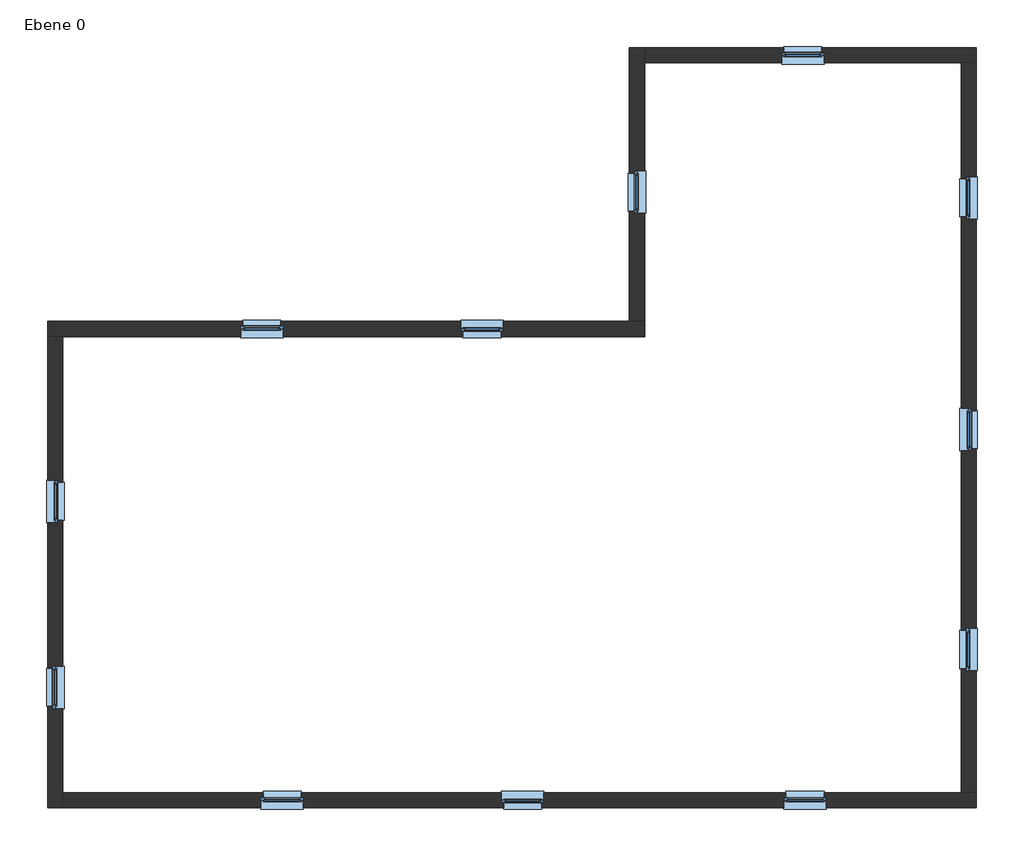
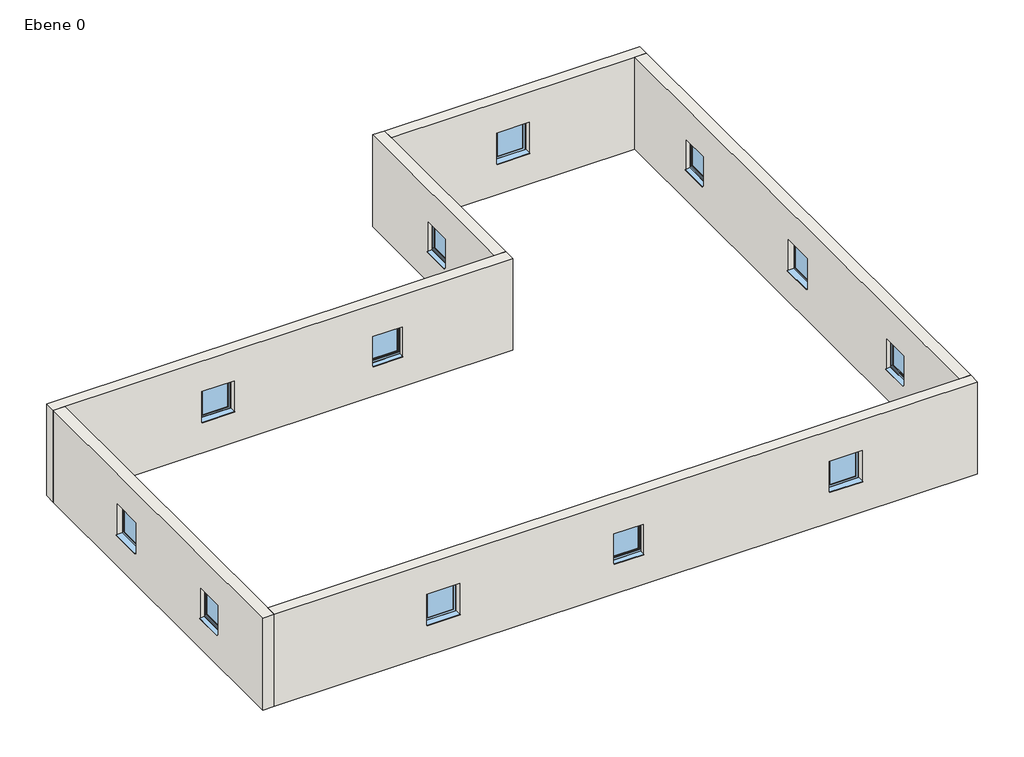
# One storey: 12 windows, 6 walls.
"""IFC4 building model written with IfcOpenShell, lengths in millimetres."""

import ifcopenshell
import ifcopenshell.guid

model = None  # the IFC model being written
_history = None  # IfcOwnerHistory: only IFC2X3 demands one
_inside = {}  # id of a spatial element -> (the spatial element, [elements in it])
_under = {}  # id of a project, library or spatial element -> (it, [spatial elements below it])
_declared = {}  # id of a project -> (the project, [libraries it declares])
_typed = {}  # id of a type object -> (the type object, [elements of that type])
_made_of = {}  # id of a material, layer set ... -> (it, [elements and type objects made of it])


def new_model(schema):
    """Start an empty IFC model of exactly this schema.

    Asked for "IFC4X3", IfcOpenShell would pick the latest addendum, in which some entities
    have other attributes; the version numbers below select the first issue.
    IFC2X3 requires an IfcOwnerHistory on every rooted entity: one is made here for all.
    """
    global model, _history
    if schema == "IFC4X3":
        model = ifcopenshell.file(schema_version=(4, 3, 0, 0))
    else:
        model = ifcopenshell.file(schema=schema)
    _inside.clear()
    _under.clear()
    _declared.clear()
    _typed.clear()
    _made_of.clear()
    _history = None
    if model.schema == "IFC2X3":
        org = make("IfcOrganization", Name="unknown")
        user = make(
            "IfcPersonAndOrganization",
            ThePerson=make("IfcPerson", FamilyName="unknown"),
            TheOrganization=org,
        )
        app = make(
            "IfcApplication",
            ApplicationDeveloper=org,
            Version="unknown",
            ApplicationFullName="unknown",
            ApplicationIdentifier="unknown",
        )
        _history = make(
            "IfcOwnerHistory",
            OwningUser=user,
            OwningApplication=app,
            ChangeAction="ADDED",
            CreationDate=0,
        )
    return model


def make(cls, **values):
    """One entity of the class cls with the attributes given. An attribute that is None is left unset."""
    return model.create_entity(
        cls, **{name: value for name, value in values.items() if value is not None}
    )


def rooted(cls, **values):
    """An entity with a GlobalId (a new one), such as an element, a storey or a relation."""
    return make(cls, GlobalId=ifcopenshell.guid.new(), OwnerHistory=_history, **values)


def si_unit(unit_type, name, prefix=None):
    """IfcSIUnit, for example si_unit("LENGTHUNIT", "METRE", prefix="MILLI")."""
    return make("IfcSIUnit", UnitType=unit_type, Prefix=prefix, Name=name)


def assignment(units):
    """IfcUnitAssignment: the units of a project."""
    return None if units is None else make("IfcUnitAssignment", Units=units)


def point(xyz):
    """IfcCartesianPoint."""
    return None if xyz is None else make("IfcCartesianPoint", Coordinates=xyz)


def direction(xyz):
    """IfcDirection."""
    return None if xyz is None else make("IfcDirection", DirectionRatios=xyz)


def frame(location, z_axis=None, x_axis=None):
    """IfcAxis2Placement3D, a coordinate frame: its origin and axes. An axis left out is left unset."""
    return make(
        "IfcAxis2Placement3D",
        Location=point(location),
        Axis=direction(z_axis),
        RefDirection=direction(x_axis),
    )


def origin():
    """The frame at (0, 0, 0) with its axes left unset."""
    return frame((0.0, 0.0, 0.0))


def place(relative_to, where):
    """IfcLocalPlacement: puts the frame where relative to a parent placement (None: the world)."""
    return make(
        "IfcLocalPlacement", PlacementRelTo=relative_to, RelativePlacement=where
    )


def context(
    kind, dimensions, precision=None, world=None, true_north=None, identifier=None
):
    """IfcGeometricRepresentationContext, for example the 3D "Model" context."""
    return make(
        "IfcGeometricRepresentationContext",
        ContextIdentifier=identifier,
        ContextType=kind,
        CoordinateSpaceDimension=dimensions,
        Precision=precision,
        WorldCoordinateSystem=world,
        TrueNorth=true_north,
    )


def project(units=None, contexts=None):
    """IfcProject with its units and contexts."""
    return rooted(
        "IfcProject",
        Name="project",
        RepresentationContexts=contexts,
        UnitsInContext=assignment(units),
    )


def spatial(cls, under=None, at=None, **own):
    """A site, building, storey or space (cls), placed at a placement, below another one or the project."""
    s = rooted(cls, ObjectPlacement=at, **own)
    if under is not None:
        _under.setdefault(under.id(), (under, []))[1].append(s)
    return s


def polyline(points):
    """IfcPolyline through the points."""
    return make("IfcPolyline", Points=[point(p) for p in points])


def outline(outer, holes=None, kind="AREA"):
    """IfcArbitraryClosedProfileDef: a profile drawn as a closed curve; with holes, ...WithVoids."""
    if holes is None:
        return make("IfcArbitraryClosedProfileDef", ProfileType=kind, OuterCurve=outer)
    return make(
        "IfcArbitraryProfileDefWithVoids",
        ProfileType=kind,
        OuterCurve=outer,
        InnerCurves=holes,
    )


def extrude(swept, where, along, depth):
    """IfcExtrudedAreaSolid: the profile swept, set in the frame where, extruded along a direction by depth."""
    return make(
        "IfcExtrudedAreaSolid",
        SweptArea=swept,
        Position=where,
        ExtrudedDirection=direction(along),
        Depth=depth,
    )


def faces_of(points, faces, orient=None, outer=None):
    """IfcFace entities. A face is a list of loops; a loop is a list of indices into points, from 0.

    orient and outer hold one flag for each loop. By default every Orientation is true, the
    first loop of a face is its IfcFaceOuterBound and the others are IfcFaceBound.
    """
    made = []
    for i, loops in enumerate(faces):
        bounds = []
        for j, loop in enumerate(loops):
            is_outer = j == 0 if outer is None else outer[i][j]
            bounds.append(
                make(
                    "IfcFaceOuterBound" if is_outer else "IfcFaceBound",
                    Bound=make("IfcPolyLoop", Polygon=[points[k] for k in loop]),
                    Orientation=True if orient is None else orient[i][j],
                )
            )
        made.append(make("IfcFace", Bounds=bounds))
    return made


def faceted_brep(points, faces, orient=None, outer=None, voids=None):
    """IfcFacetedBrep: a solid bounded by flat faces; with voids (closed shells), ...WithVoids."""
    shared = [point(p) for p in points]
    hull = make("IfcClosedShell", CfsFaces=faces_of(shared, faces, orient, outer))
    if voids is None:
        return make("IfcFacetedBrep", Outer=hull)
    return make(
        "IfcFacetedBrepWithVoids",
        Outer=hull,
        Voids=[
            make(cls, CfsFaces=faces_of(shared, fs, o, b)) for cls, fs, o, b in voids
        ],
    )


def shape(context_of_items, identifier, shape_type, items):
    """IfcShapeRepresentation: the items that make up one representation, for example the "Body"."""
    return make(
        "IfcShapeRepresentation",
        ContextOfItems=context_of_items,
        RepresentationIdentifier=identifier,
        RepresentationType=shape_type,
        Items=items,
    )


def source(mapping_origin, context_of_items, identifier, shape_type, items):
    """IfcRepresentationMap: a shape defined once, which mapped items show again and again."""
    return make(
        "IfcRepresentationMap",
        MappingOrigin=mapping_origin,
        MappedRepresentation=shape(context_of_items, identifier, shape_type, items),
    )


def transform(
    local_origin,
    x_axis=None,
    y_axis=None,
    z_axis=None,
    scale=None,
    scale2=None,
    scale3=None,
    uniform=True,
):
    """IfcCartesianTransformationOperator3D, or its non-uniform kind. x_axis, y_axis, z_axis: its Axis1, 2, 3."""
    if uniform:
        return make(
            "IfcCartesianTransformationOperator3D",
            Axis1=direction(x_axis),
            Axis2=direction(y_axis),
            LocalOrigin=point(local_origin),
            Scale=scale,
            Axis3=direction(z_axis),
        )
    return make(
        "IfcCartesianTransformationOperator3DnonUniform",
        Axis1=direction(x_axis),
        Axis2=direction(y_axis),
        LocalOrigin=point(local_origin),
        Scale=scale,
        Axis3=direction(z_axis),
        Scale2=scale2,
        Scale3=scale3,
    )


def mapped(mapping_source, mapping_target):
    """IfcMappedItem: shows the shape of a source again, moved by a transform."""
    return make(
        "IfcMappedItem", MappingSource=mapping_source, MappingTarget=mapping_target
    )


def made_of(thing, what):
    """Note that an element or type object is made of a material, layer set ...; save() writes the relation."""
    if what is not None:
        _made_of.setdefault(what.id(), (what, []))[1].append(thing)
    return thing


def element(
    cls,
    number,
    at=None,
    inside=None,
    cuts=None,
    type_object=None,
    material=None,
    context=None,
    identifier="Body",
    shape_type=None,
    held_by="IfcProductDefinitionShape",
    body=None,
    shapes=None,
    **own,
):
    """One element of the class cls, such as IfcWall. Its Tag is "e" and its number.

    at: its placement. inside: the storey or other place that contains it. cuts: it is an
    opening in that element (IfcRelVoidsElement). A single representation is given by context,
    identifier, shape_type and body (its items); several are given by shapes. held_by: the class
    of the entity that holds the representations. save() writes the other relations.
    """
    e = rooted(cls, Tag="e%d" % number, ObjectPlacement=at, **own)
    if body is not None:
        shapes = [shape(context, identifier, shape_type, body)]
    if shapes is not None:
        e.Representation = make(held_by, Representations=shapes)
    if inside is not None:
        _inside.setdefault(inside.id(), (inside, []))[1].append(e)
    if cuts is not None:
        rooted(
            "IfcRelVoidsElement", RelatingBuildingElement=cuts, RelatedOpeningElement=e
        )
    if type_object is not None:
        _typed.setdefault(type_object.id(), (type_object, []))[1].append(e)
    return made_of(e, material)


def aggregate(whole, parts):
    """IfcRelAggregates: a whole, such as a stair, and the parts it consists of."""
    return rooted("IfcRelAggregates", RelatingObject=whole, RelatedObjects=parts)


def save(model, path):
    """Write the relations noted so far, then the file.

    IfcRelAggregates (storeys below a building ...), IfcRelContainedInSpatialStructure (elements
    in a storey), IfcRelDefinesByType, IfcRelAssociatesMaterial and IfcRelDeclares: one each for
    every whole, place, type object, material and project.
    """
    for whole, parts in _under.values():
        aggregate(whole, parts)
    for where, things in _inside.values():
        rooted(
            "IfcRelContainedInSpatialStructure",
            RelatedElements=things,
            RelatingStructure=where,
        )
    for kind, things in _typed.values():
        rooted("IfcRelDefinesByType", RelatedObjects=things, RelatingType=kind)
    for what, things in _made_of.values():
        rooted("IfcRelAssociatesMaterial", RelatedObjects=things, RelatingMaterial=what)
    for by, libraries in _declared.values():
        rooted("IfcRelDeclares", RelatingContext=by, RelatedDefinitions=libraries)
    model.write(path)


def window_1_01_x_1_01_b7243dc8(model_context):
    return source(origin(), model_context, "Body", "SolidModel", [
        extrude(outline(polyline([(-525.0, -210.0), (-525.0, 0.0), (485.0, 0.0), (485.0, -210.0), (-525.0, -210.0)])), frame((0.0, 0.0, 1005.0), z_axis=(0.0, 0.0, 1.0), x_axis=(1.0, 0.0, 0.0)), (0.0, 0.0, 1.0), 15.0),
        extrude(outline(polyline([(375.0, -15.0), (-415.0, -15.0), (-415.0, 15.0), (375.0, 15.0), (375.0, -15.0)])), frame((0.0, 0.0, 1110.0), z_axis=(0.0, 0.0, 1.0), x_axis=(1.0, 0.0, 0.0)), (0.0, 0.0, 1.0), 790.0),
        extrude(outline(polyline([(70.0221543, 1020.0), (210.0, 1000.0), (210.0, 990.0), (208.0, 990.0), (208.0, 998.3604634), (69.8240723, 1018.0), (60.0, 1018.0), (60.0, 1020.0), (70.0221543, 1020.0)])), frame((-475.0, 0.0, 0.0), z_axis=(1.0, 0.0, 0.0), x_axis=(0.0, 1.0, 0.0)), (0.0, 0.0, 1.0), 910.0),
        extrude(outline(polyline([(2010.0, 485.0), (2010.0, -525.0), (1000.0, -525.0), (1000.0, 485.0), (2010.0, 485.0)]), holes=[polyline([(1930.0, 405.0), (1080.0, 405.0), (1080.0, -445.0), (1930.0, -445.0), (1930.0, 405.0)])]), frame((0.0, 0.0, 0.0), z_axis=(0.0, 1.0, 0.0), x_axis=(0.0, 0.0, 1.0)), (0.0, 0.0, 1.0), 60.0),
        faceted_brep([(435.0, 0.0, 1960.0), (435.0, -30.0, 1960.0), (435.0, -30.0, 1050.0), (435.0, 0.0, 1050.0), (-475.0, -30.0, 1960.0), (-475.0, -30.0, 1050.0), (375.0, -30.0, 1110.0), (-415.0, -30.0, 1110.0), (-415.0, -30.0, 1900.0), (375.0, -30.0, 1900.0), (-475.0, 0.0, 1050.0), (-475.0, 0.0, 1960.0), (405.0, 0.0, 1930.0), (-445.0, 0.0, 1930.0), (-445.0, 0.0, 1080.0), (405.0, 0.0, 1080.0), (405.0, 30.0, 1930.0), (405.0, 30.0, 1080.0), (-445.0, 30.0, 1080.0), (-445.0, 30.0, 1930.0), (375.0, 30.0, 1900.0), (-415.0, 30.0, 1900.0), (-415.0, 30.0, 1110.0), (375.0, 30.0, 1110.0)], [[[0, 1, 2, 3]], [[1, 4, 5, 2], [6, 7, 8, 9]], [[3, 2, 5, 10]], [[3, 10, 11, 0], [12, 13, 14, 15]], [[16, 12, 15, 17]], [[17, 15, 14, 18]], [[17, 18, 19, 16], [20, 21, 22, 23]], [[9, 20, 23, 6]], [[6, 23, 22, 7]], [[10, 5, 4, 11]], [[18, 14, 13, 19]], [[7, 22, 21, 8]], [[11, 4, 1, 0]], [[19, 13, 12, 16]], [[8, 21, 20, 9]]]),
    ])


model = new_model("IFC4")

# Units and contexts
model_context = context("Model", 3, world=origin())
ifc_project = project(units=[si_unit("LENGTHUNIT", "METRE", prefix="MILLI")], contexts=[model_context])

# Site, building, storey
site = spatial("IfcSite", under=ifc_project)
building = spatial("IfcBuilding", under=site)
storey = spatial("IfcBuildingStorey", under=building, Name="Ebene 0", Elevation=0.0)

# Walls
placement = place(None, origin())
element("IfcWall", 1, ObjectType="MW 24.0 WD 12.0", at=placement, inside=storey, context=model_context, shape_type="Brep", body=[
    faceted_brep([(-13369.6797169, 6985.6067473, 0.0), (-13009.6797169, 6985.6067473, 0.0), (810.3202831, 6985.6067473, 0.0), (810.3202831, 6985.6067473, 3000.0), (-13009.6797169, 6985.6067473, 3000.0), (-13369.6797169, 6985.6067473, 3000.0), (-3509.6797169, 6985.6067473, 1960.0), (-2599.6797169, 6985.6067473, 1960.0), (-2599.6797169, 6985.6067473, 1000.0), (-3509.6797169, 6985.6067473, 1000.0), (-7779.6797169, 6985.6067473, 1000.0), (-8789.6797169, 6985.6067473, 1000.0), (-8789.6797169, 6985.6067473, 2010.0), (-7779.6797169, 6985.6067473, 2010.0), (-13369.6797169, 7345.6067473, 0.0), (-13369.6797169, 7345.6067473, 3000.0), (450.3202831, 7345.6067473, 3000.0), (810.3202831, 7345.6067473, 3000.0), (810.3202831, 7345.6067473, 0.0), (450.3202831, 7345.6067473, 0.0), (-3559.6797169, 7345.6067473, 1000.0), (-2549.6797169, 7345.6067473, 1000.0), (-2549.6797169, 7345.6067473, 2010.0), (-3559.6797169, 7345.6067473, 2010.0), (-7829.6797169, 7345.6067473, 1960.0), (-8739.6797169, 7345.6067473, 1960.0), (-8739.6797169, 7345.6067473, 1000.0), (-7829.6797169, 7345.6067473, 1000.0), (-3509.6797169, 7105.6067473, 1960.0), (-2599.6797169, 7105.6067473, 1960.0), (-2599.6797169, 7105.6067473, 1000.0), (-3509.6797169, 7105.6067473, 1000.0), (-2549.6797169, 7105.6067473, 1000.0), (-3559.6797169, 7105.6067473, 1000.0), (-2549.6797169, 7105.6067473, 2010.0), (-3559.6797169, 7105.6067473, 2010.0), (-7829.6797169, 7225.6067473, 1960.0), (-8739.6797169, 7225.6067473, 1960.0), (-8739.6797169, 7225.6067473, 1000.0), (-7829.6797169, 7225.6067473, 1000.0), (-8789.6797169, 7225.6067473, 1000.0), (-7779.6797169, 7225.6067473, 1000.0), (-8789.6797169, 7225.6067473, 2010.0), (-7779.6797169, 7225.6067473, 2010.0)], [[[0, 1, 2, 3, 4, 5], [6, 7, 8, 9], [10, 11, 12, 13]], [[14, 15, 16, 17, 18, 19], [20, 21, 22, 23], [24, 25, 26, 27]], [[2, 1, 0, 14, 19, 18]], [[5, 4, 3, 17, 16, 15]], [[0, 5, 15, 14]], [[3, 2, 18, 17]], [[6, 28, 29, 7]], [[7, 29, 30, 8]], [[28, 6, 9, 31]], [[8, 30, 32, 21, 20, 33, 31, 9]], [[34, 35, 23, 22]], [[35, 33, 20, 23]], [[35, 34, 32, 30, 29, 28, 31, 33]], [[32, 34, 22, 21]], [[24, 36, 37, 25]], [[25, 37, 38, 26]], [[36, 24, 27, 39]], [[26, 38, 40, 11, 10, 41, 39, 27]], [[42, 43, 13, 12]], [[43, 41, 10, 13]], [[43, 42, 40, 38, 37, 36, 39, 41]], [[40, 42, 12, 11]]]),
])
element("IfcWall", 2, ObjectType="MW 24.0 WD 12.0", at=placement, inside=storey, context=model_context, shape_type="Brep", body=[
    faceted_brep([(-13009.6797169, -4214.3932527, 0.0), (-13009.6797169, -3854.3932527, 0.0), (-13009.6797169, 6985.6067473, 0.0), (-13009.6797169, 6985.6067473, 3000.0), (-13009.6797169, -3854.3932527, 3000.0), (-13009.6797169, -4214.3932527, 3000.0), (-13009.6797169, -844.3932527, 1000.0), (-13009.6797169, -1854.3932527, 1000.0), (-13009.6797169, -1854.3932527, 2010.0), (-13009.6797169, -844.3932527, 2010.0), (-13009.6797169, 2615.6067473, 1960.0), (-13009.6797169, 3525.6067473, 1960.0), (-13009.6797169, 3525.6067473, 1000.0), (-13009.6797169, 2615.6067473, 1000.0), (-13369.6797169, -4214.3932527, 0.0), (-13369.6797169, -4214.3932527, 3000.0), (-13369.6797169, 6985.6067473, 3000.0), (-13369.6797169, 6985.6067473, 0.0), (-13369.6797169, -894.3932527, 1960.0), (-13369.6797169, -1804.3932527, 1960.0), (-13369.6797169, -1804.3932527, 1000.0), (-13369.6797169, -894.3932527, 1000.0), (-13369.6797169, 2565.6067473, 1000.0), (-13369.6797169, 3575.6067473, 1000.0), (-13369.6797169, 3575.6067473, 2010.0), (-13369.6797169, 2565.6067473, 2010.0), (-13249.6797169, -894.3932527, 1960.0), (-13249.6797169, -1804.3932527, 1960.0), (-13249.6797169, -1804.3932527, 1000.0), (-13249.6797169, -894.3932527, 1000.0), (-13249.6797169, -1854.3932527, 1000.0), (-13249.6797169, -844.3932527, 1000.0), (-13249.6797169, -1854.3932527, 2010.0), (-13249.6797169, -844.3932527, 2010.0), (-13129.6797169, 2615.6067473, 1960.0), (-13129.6797169, 3525.6067473, 1960.0), (-13129.6797169, 3525.6067473, 1000.0), (-13129.6797169, 2615.6067473, 1000.0), (-13129.6797169, 3575.6067473, 1000.0), (-13129.6797169, 2565.6067473, 1000.0), (-13129.6797169, 3575.6067473, 2010.0), (-13129.6797169, 2565.6067473, 2010.0)], [[[0, 1, 2, 3, 4, 5], [6, 7, 8, 9], [10, 11, 12, 13]], [[14, 15, 16, 17], [18, 19, 20, 21], [22, 23, 24, 25]], [[2, 1, 0, 14, 17]], [[5, 4, 3, 16, 15]], [[0, 5, 15, 14]], [[3, 2, 17, 16]], [[18, 26, 27, 19]], [[19, 27, 28, 20]], [[26, 18, 21, 29]], [[20, 28, 30, 7, 6, 31, 29, 21]], [[32, 33, 9, 8]], [[33, 31, 6, 9]], [[33, 32, 30, 28, 27, 26, 29, 31]], [[30, 32, 8, 7]], [[10, 34, 35, 11]], [[11, 35, 36, 12]], [[34, 10, 13, 37]], [[12, 36, 38, 23, 22, 39, 37, 13]], [[40, 41, 25, 24]], [[41, 39, 22, 25]], [[41, 40, 38, 36, 35, 34, 37, 39]], [[38, 40, 24, 23]]]),
])
element("IfcWall", 3, ObjectType="MW 24.0 WD 12.0", at=placement, inside=storey, context=model_context, shape_type="Brep", body=[
    faceted_brep([(8690.3202831, -3854.3932527, 0.0), (8330.3202831, -3854.3932527, 0.0), (-13009.6797169, -3854.3932527, 0.0), (-13009.6797169, -3854.3932527, 3000.0), (8330.3202831, -3854.3932527, 3000.0), (8690.3202831, -3854.3932527, 3000.0), (5080.3202831, -3854.3932527, 1960.0), (4170.3202831, -3854.3932527, 1960.0), (4170.3202831, -3854.3932527, 1000.0), (5080.3202831, -3854.3932527, 1000.0), (-2589.6797169, -3854.3932527, 1000.0), (-1579.6797169, -3854.3932527, 1000.0), (-1579.6797169, -3854.3932527, 2010.0), (-2589.6797169, -3854.3932527, 2010.0), (-7344.6797169, -3854.3932527, 1960.0), (-8254.6797169, -3854.3932527, 1960.0), (-8254.6797169, -3854.3932527, 1000.0), (-7344.6797169, -3854.3932527, 1000.0), (8690.3202831, -4214.3932527, 0.0), (8690.3202831, -4214.3932527, 3000.0), (-13009.6797169, -4214.3932527, 3000.0), (-13009.6797169, -4214.3932527, 0.0), (5130.3202831, -4214.3932527, 1000.0), (4120.3202831, -4214.3932527, 1000.0), (4120.3202831, -4214.3932527, 2010.0), (5130.3202831, -4214.3932527, 2010.0), (-2539.6797169, -4214.3932527, 1960.0), (-1629.6797169, -4214.3932527, 1960.0), (-1629.6797169, -4214.3932527, 1000.0), (-2539.6797169, -4214.3932527, 1000.0), (-7294.6797169, -4214.3932527, 1000.0), (-8304.6797169, -4214.3932527, 1000.0), (-8304.6797169, -4214.3932527, 2010.0), (-7294.6797169, -4214.3932527, 2010.0), (5080.3202831, -3974.3932527, 1960.0), (4170.3202831, -3974.3932527, 1960.0), (4170.3202831, -3974.3932527, 1000.0), (5080.3202831, -3974.3932527, 1000.0), (4120.3202831, -3974.3932527, 1000.0), (5130.3202831, -3974.3932527, 1000.0), (4120.3202831, -3974.3932527, 2010.0), (5130.3202831, -3974.3932527, 2010.0), (-2539.6797169, -4094.3932527, 1960.0), (-1629.6797169, -4094.3932527, 1960.0), (-1629.6797169, -4094.3932527, 1000.0), (-2539.6797169, -4094.3932527, 1000.0), (-1579.6797169, -4094.3932527, 1000.0), (-2589.6797169, -4094.3932527, 1000.0), (-1579.6797169, -4094.3932527, 2010.0), (-2589.6797169, -4094.3932527, 2010.0), (-7344.6797169, -3974.3932527, 1960.0), (-8254.6797169, -3974.3932527, 1960.0), (-8254.6797169, -3974.3932527, 1000.0), (-7344.6797169, -3974.3932527, 1000.0), (-8304.6797169, -3974.3932527, 1000.0), (-7294.6797169, -3974.3932527, 1000.0), (-8304.6797169, -3974.3932527, 2010.0), (-7294.6797169, -3974.3932527, 2010.0)], [[[0, 1, 2, 3, 4, 5], [6, 7, 8, 9], [10, 11, 12, 13], [14, 15, 16, 17]], [[18, 19, 20, 21], [22, 23, 24, 25], [26, 27, 28, 29], [30, 31, 32, 33]], [[2, 1, 0, 18, 21]], [[5, 4, 3, 20, 19]], [[0, 5, 19, 18]], [[3, 2, 21, 20]], [[6, 34, 35, 7]], [[7, 35, 36, 8]], [[34, 6, 9, 37]], [[8, 36, 38, 23, 22, 39, 37, 9]], [[40, 41, 25, 24]], [[41, 39, 22, 25]], [[41, 40, 38, 36, 35, 34, 37, 39]], [[38, 40, 24, 23]], [[26, 42, 43, 27]], [[27, 43, 44, 28]], [[42, 26, 29, 45]], [[28, 44, 46, 11, 10, 47, 45, 29]], [[48, 49, 13, 12]], [[49, 47, 10, 13]], [[49, 48, 46, 44, 43, 42, 45, 47]], [[46, 48, 12, 11]], [[14, 50, 51, 15]], [[15, 51, 52, 16]], [[50, 14, 17, 53]], [[16, 52, 54, 31, 30, 55, 53, 17]], [[56, 57, 33, 32]], [[57, 55, 30, 33]], [[57, 56, 54, 52, 51, 50, 53, 55]], [[54, 56, 32, 31]]]),
])
element("IfcWall", 4, ObjectType="MW 24.0 WD 12.0", at=placement, inside=storey, context=model_context, shape_type="Brep", body=[
    faceted_brep([(8330.3202831, 13485.6067473, 0.0), (8330.3202831, -3854.3932527, 0.0), (8330.3202831, -3854.3932527, 3000.0), (8330.3202831, 13485.6067473, 3000.0), (8330.3202831, 10735.6067473, 1960.0), (8330.3202831, 9825.6067473, 1960.0), (8330.3202831, 9825.6067473, 1000.0), (8330.3202831, 10735.6067473, 1000.0), (8330.3202831, 4265.6067473, 1000.0), (8330.3202831, 5275.6067473, 1000.0), (8330.3202831, 5275.6067473, 2010.0), (8330.3202831, 4265.6067473, 2010.0), (8330.3202831, 5.6067473, 1960.0), (8330.3202831, -904.3932527, 1960.0), (8330.3202831, -904.3932527, 1000.0), (8330.3202831, 5.6067473, 1000.0), (8690.3202831, 13485.6067473, 0.0), (8690.3202831, 13485.6067473, 3000.0), (8690.3202831, -3854.3932527, 3000.0), (8690.3202831, -3854.3932527, 0.0), (8690.3202831, 10785.6067473, 1000.0), (8690.3202831, 9775.6067473, 1000.0), (8690.3202831, 9775.6067473, 2010.0), (8690.3202831, 10785.6067473, 2010.0), (8690.3202831, 4315.6067473, 1960.0), (8690.3202831, 5225.6067473, 1960.0), (8690.3202831, 5225.6067473, 1000.0), (8690.3202831, 4315.6067473, 1000.0), (8690.3202831, 55.6067473, 1000.0), (8690.3202831, -954.3932527, 1000.0), (8690.3202831, -954.3932527, 2010.0), (8690.3202831, 55.6067473, 2010.0), (8450.3202831, 10735.6067473, 1960.0), (8450.3202831, 9825.6067473, 1960.0), (8450.3202831, 9825.6067473, 1000.0), (8450.3202831, 10735.6067473, 1000.0), (8450.3202831, 9775.6067473, 1000.0), (8450.3202831, 10785.6067473, 1000.0), (8450.3202831, 9775.6067473, 2010.0), (8450.3202831, 10785.6067473, 2010.0), (8570.3202831, 4315.6067473, 1960.0), (8570.3202831, 5225.6067473, 1960.0), (8570.3202831, 5225.6067473, 1000.0), (8570.3202831, 4315.6067473, 1000.0), (8570.3202831, 5275.6067473, 1000.0), (8570.3202831, 4265.6067473, 1000.0), (8570.3202831, 5275.6067473, 2010.0), (8570.3202831, 4265.6067473, 2010.0), (8450.3202831, 5.6067473, 1960.0), (8450.3202831, -904.3932527, 1960.0), (8450.3202831, -904.3932527, 1000.0), (8450.3202831, 5.6067473, 1000.0), (8450.3202831, -954.3932527, 1000.0), (8450.3202831, 55.6067473, 1000.0), (8450.3202831, -954.3932527, 2010.0), (8450.3202831, 55.6067473, 2010.0)], [[[0, 1, 2, 3], [4, 5, 6, 7], [8, 9, 10, 11], [12, 13, 14, 15]], [[16, 17, 18, 19], [20, 21, 22, 23], [24, 25, 26, 27], [28, 29, 30, 31]], [[1, 0, 16, 19]], [[3, 2, 18, 17]], [[2, 1, 19, 18]], [[0, 3, 17, 16]], [[4, 32, 33, 5]], [[5, 33, 34, 6]], [[32, 4, 7, 35]], [[6, 34, 36, 21, 20, 37, 35, 7]], [[38, 39, 23, 22]], [[39, 37, 20, 23]], [[39, 38, 36, 34, 33, 32, 35, 37]], [[36, 38, 22, 21]], [[24, 40, 41, 25]], [[25, 41, 42, 26]], [[40, 24, 27, 43]], [[26, 42, 44, 9, 8, 45, 43, 27]], [[46, 47, 11, 10]], [[47, 45, 8, 11]], [[47, 46, 44, 42, 41, 40, 43, 45]], [[44, 46, 10, 9]], [[12, 48, 49, 13]], [[13, 49, 50, 14]], [[48, 12, 15, 51]], [[14, 50, 52, 29, 28, 53, 51, 15]], [[54, 55, 31, 30]], [[55, 53, 28, 31]], [[55, 54, 52, 50, 49, 48, 51, 53]], [[52, 54, 30, 29]]]),
])
element("IfcWall", 5, ObjectType="MW 24.0 WD 12.0", at=placement, inside=storey, context=model_context, shape_type="Brep", body=[
    faceted_brep([(810.3202831, 7345.6067473, 0.0), (810.3202831, 13485.6067473, 0.0), (810.3202831, 13845.6067473, 0.0), (810.3202831, 13845.6067473, 3000.0), (810.3202831, 13485.6067473, 3000.0), (810.3202831, 7345.6067473, 3000.0), (810.3202831, 10920.6067473, 1000.0), (810.3202831, 9910.6067473, 1000.0), (810.3202831, 9910.6067473, 2010.0), (810.3202831, 10920.6067473, 2010.0), (450.3202831, 7345.6067473, 0.0), (450.3202831, 7345.6067473, 3000.0), (450.3202831, 13845.6067473, 3000.0), (450.3202831, 13845.6067473, 0.0), (450.3202831, 10870.6067473, 1960.0), (450.3202831, 9960.6067473, 1960.0), (450.3202831, 9960.6067473, 1000.0), (450.3202831, 10870.6067473, 1000.0), (570.3202831, 10870.6067473, 1960.0), (570.3202831, 9960.6067473, 1960.0), (570.3202831, 9960.6067473, 1000.0), (570.3202831, 10870.6067473, 1000.0), (570.3202831, 9910.6067473, 1000.0), (570.3202831, 10920.6067473, 1000.0), (570.3202831, 9910.6067473, 2010.0), (570.3202831, 10920.6067473, 2010.0)], [[[0, 1, 2, 3, 4, 5], [6, 7, 8, 9]], [[10, 11, 12, 13], [14, 15, 16, 17]], [[2, 1, 0, 10, 13]], [[5, 4, 3, 12, 11]], [[3, 2, 13, 12]], [[0, 5, 11, 10]], [[14, 18, 19, 15]], [[15, 19, 20, 16]], [[18, 14, 17, 21]], [[16, 20, 22, 7, 6, 23, 21, 17]], [[24, 25, 9, 8]], [[25, 23, 6, 9]], [[25, 24, 22, 20, 19, 18, 21, 23]], [[22, 24, 8, 7]]]),
])
element("IfcWall", 6, ObjectType="MW 24.0 WD 12.0", at=placement, inside=storey, context=model_context, shape_type="Brep", body=[
    faceted_brep([(810.3202831, 13485.6067473, 0.0), (8330.3202831, 13485.6067473, 0.0), (8690.3202831, 13485.6067473, 0.0), (8690.3202831, 13485.6067473, 3000.0), (8330.3202831, 13485.6067473, 3000.0), (810.3202831, 13485.6067473, 3000.0), (5075.3202831, 13485.6067473, 1000.0), (4065.3202831, 13485.6067473, 1000.0), (4065.3202831, 13485.6067473, 2010.0), (5075.3202831, 13485.6067473, 2010.0), (810.3202831, 13845.6067473, 0.0), (810.3202831, 13845.6067473, 3000.0), (8690.3202831, 13845.6067473, 3000.0), (8690.3202831, 13845.6067473, 0.0), (5025.3202831, 13845.6067473, 1960.0), (4115.3202831, 13845.6067473, 1960.0), (4115.3202831, 13845.6067473, 1000.0), (5025.3202831, 13845.6067473, 1000.0), (5025.3202831, 13725.6067473, 1960.0), (4115.3202831, 13725.6067473, 1960.0), (4115.3202831, 13725.6067473, 1000.0), (5025.3202831, 13725.6067473, 1000.0), (4065.3202831, 13725.6067473, 1000.0), (5075.3202831, 13725.6067473, 1000.0), (4065.3202831, 13725.6067473, 2010.0), (5075.3202831, 13725.6067473, 2010.0)], [[[0, 1, 2, 3, 4, 5], [6, 7, 8, 9]], [[10, 11, 12, 13], [14, 15, 16, 17]], [[2, 1, 0, 10, 13]], [[5, 4, 3, 12, 11]], [[0, 5, 11, 10]], [[3, 2, 13, 12]], [[14, 18, 19, 15]], [[15, 19, 20, 16]], [[18, 14, 17, 21]], [[16, 20, 22, 7, 6, 23, 21, 17]], [[24, 25, 9, 8]], [[25, 23, 6, 9]], [[25, 24, 22, 20, 19, 18, 21, 23]], [[22, 24, 8, 7]]]),
])

# Windows
window_1_01_x_1_01_shape = window_1_01_x_1_01_b7243dc8(model_context)
element("IfcWindow", 7, ObjectType="Fenster 1-flg - Anschlag : 1.01 x 1.01", at=placement, inside=storey, context=model_context, shape_type="MappedRepresentation", body=[
    mapped(window_1_01_x_1_01_shape, transform((4590.3202831, 13665.6067473, 0.0), x_axis=(1.0, 0.0, 0.0), y_axis=(0.0, 1.0, 0.0), z_axis=(0.0, 0.0, 1.0))),
])
element("IfcWindow", 8, ObjectType="Fenster 1-flg - Anschlag : 1.01 x 1.01", at=placement, inside=storey, context=model_context, shape_type="MappedRepresentation", body=[
    mapped(window_1_01_x_1_01_shape, transform((630.3202831, 10435.6067473, 0.0), x_axis=(0.0, 1.0, 0.0), y_axis=(-1.0, 0.0, 0.0), z_axis=(0.0, 0.0, 1.0))),
])
element("IfcWindow", 9, ObjectType="Fenster 1-flg - Anschlag : 1.01 x 1.01", at=placement, inside=storey, context=model_context, shape_type="MappedRepresentation", body=[
    mapped(window_1_01_x_1_01_shape, transform((-8264.6797169, 7165.6067473, 0.0), x_axis=(1.0, 0.0, 0.0), y_axis=(0.0, 1.0, 0.0), z_axis=(0.0, 0.0, 1.0))),
])
element("IfcWindow", 10, ObjectType="Fenster 1-flg - Anschlag : 1.01 x 1.01", at=placement, inside=storey, context=model_context, shape_type="MappedRepresentation", body=[
    mapped(window_1_01_x_1_01_shape, transform((8510.3202831, 4750.6067473, 0.0), x_axis=(0.0, -1.0, 0.0), y_axis=(1.0, 0.0, 0.0), z_axis=(0.0, 0.0, 1.0))),
])
element("IfcWindow", 11, ObjectType="Fenster 1-flg - Anschlag : 1.01 x 1.01", at=placement, inside=storey, context=model_context, shape_type="MappedRepresentation", body=[
    mapped(window_1_01_x_1_01_shape, transform((-2104.6797169, -4034.3932527, 0.0), x_axis=(-1.0, 0.0, 0.0), y_axis=(0.0, -1.0, 0.0), z_axis=(0.0, 0.0, 1.0))),
])
element("IfcWindow", 12, ObjectType="Fenster 1-flg - Anschlag : 1.01 x 1.01", at=placement, inside=storey, context=model_context, shape_type="MappedRepresentation", body=[
    mapped(window_1_01_x_1_01_shape, transform((-13189.6797169, -1329.3932527, 0.0), x_axis=(0.0, 1.0, 0.0), y_axis=(-1.0, 0.0, 0.0), z_axis=(0.0, 0.0, 1.0))),
])
element("IfcWindow", 13, ObjectType="Fenster 1-flg - Anschlag : 1.01 x 1.01", at=placement, inside=storey, context=model_context, shape_type="MappedRepresentation", body=[
    mapped(window_1_01_x_1_01_shape, transform((-3074.6797169, 7165.6067473, 0.0), x_axis=(-1.0, 0.0, 0.0), y_axis=(0.0, -1.0, 0.0), z_axis=(0.0, 0.0, 1.0))),
])
element("IfcWindow", 14, ObjectType="Fenster 1-flg - Anschlag : 1.01 x 1.01", at=placement, inside=storey, context=model_context, shape_type="MappedRepresentation", body=[
    mapped(window_1_01_x_1_01_shape, transform((8510.3202831, 10300.6067473, 0.0), x_axis=(0.0, 1.0, 0.0), y_axis=(-1.0, 0.0, 0.0), z_axis=(0.0, 0.0, 1.0))),
])
element("IfcWindow", 15, ObjectType="Fenster 1-flg - Anschlag : 1.01 x 1.01", at=placement, inside=storey, context=model_context, shape_type="MappedRepresentation", body=[
    mapped(window_1_01_x_1_01_shape, transform((8510.3202831, -429.3932527, 0.0), x_axis=(0.0, 1.0, 0.0), y_axis=(-1.0, 0.0, 0.0), z_axis=(0.0, 0.0, 1.0))),
])
element("IfcWindow", 16, ObjectType="Fenster 1-flg - Anschlag : 1.01 x 1.01", at=placement, inside=storey, context=model_context, shape_type="MappedRepresentation", body=[
    mapped(window_1_01_x_1_01_shape, transform((4645.3202831, -4034.3932527, 0.0), x_axis=(1.0, 0.0, 0.0), y_axis=(0.0, 1.0, 0.0), z_axis=(0.0, 0.0, 1.0))),
])
element("IfcWindow", 17, ObjectType="Fenster 1-flg - Anschlag : 1.01 x 1.01", at=placement, inside=storey, context=model_context, shape_type="MappedRepresentation", body=[
    mapped(window_1_01_x_1_01_shape, transform((-7779.6797169, -4034.3932527, 0.0), x_axis=(1.0, 0.0, 0.0), y_axis=(0.0, 1.0, 0.0), z_axis=(0.0, 0.0, 1.0))),
])
element("IfcWindow", 18, ObjectType="Fenster 1-flg - Anschlag : 1.01 x 1.01", at=placement, inside=storey, context=model_context, shape_type="MappedRepresentation", body=[
    mapped(window_1_01_x_1_01_shape, transform((-13189.6797169, 3050.6067473, 0.0), x_axis=(0.0, -1.0, 0.0), y_axis=(1.0, 0.0, 0.0), z_axis=(0.0, 0.0, 1.0))),
])

save(model, "model.ifc")

# Revit data of these elements
# Project information
#   Projektausgabedatum = "Projekt Datum"
#   Projektstatus = "Projektstatus"
#   Kundenname = "Bauherr"
#   Projektadresse = "Projektadresse"
#   Projektname = "Projektname"
#   Projektnummer = "Projektnummer"
#   Verfasser Firma 1 = "Firma 1"
#   Verfasser Firma 2 = "Firma 2"
#   Verfasser PLZ Ort = "PLZ Ort"
#   Verfasser Strasse = "Strasse"
#   Verfasser Telefon = "Telefon"
#   Verfasser Telefax = "Telefax"
#   Verfasser eMail = "E-Mail"
# Type "MW 24.0 WD 12.0"
#   Type Comments = "Mehrschaliges Mauerwerk"
#   Description = "Mauerwerk 24.0 cm, Wärmedämmung 12.0 cm"
#   Width = 0.360 m
#   Layers, outside or top first: 0.120 m "Wärmedämmung - Hart" (function 3); 0.240 m "Mauerwerk - Ziegel, verputzt" (function 1)
# Type "Fenster 1-flg - Anschlag : 1.01 x 1.01"
#   Type Mark = "47"
#   Operation = "SinglePanel"
#   Keynote = "16.05.01"
#   Construction Type Id = "GSP4R"
#   Analytic Construction = "1/8 Zoll Pilkington-Verglasung einfach"
#   Visual Light Transmittance = 0.9
#   Thermal Resistance (R) = 0.1491 (m²·K)/W
#   Solar Heat Gain Coefficient = 0.86
#   Anschlagsbreite seitlich = 0.050 m
#   Rough Width = 1.010 m
#   Rough Height = 1.010 m
#   Heat Transfer Coefficient (U) = 6.7069 W/(m²·K)
#   Rahmentiefe = 0.060 m
#   Rahmenhöhe unten = 0.080 m
#   Rahmenhöhe oben = 0.080 m
#   Rahmenbreite = 0.080 m
#   Height = 1.010 m
#   Flügeltiefe = 0.060 m
#   Flügelbreite = 0.060 m
#   Einbautiefe (von außen) [instance default] = 0.120 m
#   Width = 1.010 m
#   Anschlagsbreite oben = 0.050 m
#   Klappflügel [instance default] = no
#   Öffnungsrichtung oben [instance default] = yes
#   Öffnungsrichtung in Draufsicht anzeigen [instance default] = no
#   Drehflügel [instance default] = yes
#   Rahmen [instance default] = none
#   Glas [instance default] = none
#   Flügel [instance default] = none
#   Fensterbank innen [instance default] = none
#   Fensterbank außen [instance default] = none
#   Wall Closure = (empty or 0)
# Elements 1, 4 (IfcWall, "MW 24.0 WD 12.0")
#   Top Offset = 0.000 m
#   Base Offset = 0.000 m
#   wall height = 3.000 m
#   Phase Created = Phase 1
#   Base Constraint = Ebene 0
#   Top Constraint = Ebene 1
#   Materials on its faces: "Standard - Wand", "Mauerwerk - Ziegel, verputzt", "Wärmedämmung - Hart"
# Elements 2, 3, 5, 6 (IfcWall, "MW 24.0 WD 12.0")
#   Top Offset = 0.000 m
#   Base Offset = 0.000 m
#   wall height = 3.000 m
#   Phase Created = Phase 1
#   Base Constraint = Ebene 0
#   Top Constraint = Ebene 1
#   Materials on its faces: "Standard - Wand", "Wärmedämmung - Hart", "Mauerwerk - Ziegel, verputzt"
# Element 7 (IfcWindow, "Fenster 1-flg - Anschlag : 1.01 x 1.01")
#   Mark = "1"
#   Einbautiefe (von außen) = 0.120 m
#   Öffnungsrichtung oben = yes
#   Öffnungsrichtung in Draufsicht anzeigen = no
#   Klappflügel = no
#   Drehflügel = yes
#   Rahmen = none
#   Glas = none
#   Flügel = none
#   Fensterbank innen = none
#   Fensterbank außen = none
#   Phase Created = Phase 1
#   Materials on its faces: "Kunststoff - Weiß", "Holz - Birke", "Glas"
# Element 8 (IfcWindow, "Fenster 1-flg - Anschlag : 1.01 x 1.01")
#   Mark = "2"
#   Einbautiefe (von außen) = 0.120 m
#   Öffnungsrichtung oben = yes
#   Öffnungsrichtung in Draufsicht anzeigen = no
#   Klappflügel = no
#   Drehflügel = yes
#   Rahmen = none
#   Glas = none
#   Flügel = none
#   Fensterbank innen = none
#   Fensterbank außen = none
#   Phase Created = Phase 1
#   Materials on its faces: "Kunststoff - Weiß", "Holz - Birke", "Glas"
# Element 9 (IfcWindow, "Fenster 1-flg - Anschlag : 1.01 x 1.01")
#   Mark = "4"
#   Einbautiefe (von außen) = 0.120 m
#   Öffnungsrichtung oben = yes
#   Öffnungsrichtung in Draufsicht anzeigen = no
#   Klappflügel = no
#   Drehflügel = yes
#   Rahmen = none
#   Glas = none
#   Flügel = none
#   Fensterbank innen = none
#   Fensterbank außen = none
#   Phase Created = Phase 1
#   Materials on its faces: "Kunststoff - Weiß", "Holz - Birke", "Glas"
# Element 10 (IfcWindow, "Fenster 1-flg - Anschlag : 1.01 x 1.01")
#   Mark = "6"
#   Einbautiefe (von außen) = 0.120 m
#   Öffnungsrichtung oben = yes
#   Öffnungsrichtung in Draufsicht anzeigen = no
#   Klappflügel = no
#   Drehflügel = yes
#   Rahmen = none
#   Glas = none
#   Flügel = none
#   Fensterbank innen = none
#   Fensterbank außen = none
#   Phase Created = Phase 1
#   Materials on its faces: "Kunststoff - Weiß", "Holz - Birke", "Glas"
# Element 11 (IfcWindow, "Fenster 1-flg - Anschlag : 1.01 x 1.01")
#   Mark = "9"
#   Einbautiefe (von außen) = 0.120 m
#   Öffnungsrichtung oben = yes
#   Öffnungsrichtung in Draufsicht anzeigen = no
#   Klappflügel = no
#   Drehflügel = yes
#   Rahmen = none
#   Glas = none
#   Flügel = none
#   Fensterbank innen = none
#   Fensterbank außen = none
#   Phase Created = Phase 1
#   Materials on its faces: "Kunststoff - Weiß", "Holz - Birke", "Glas"
# Element 12 (IfcWindow, "Fenster 1-flg - Anschlag : 1.01 x 1.01")
#   Mark = "11"
#   Einbautiefe (von außen) = 0.120 m
#   Öffnungsrichtung oben = yes
#   Öffnungsrichtung in Draufsicht anzeigen = no
#   Klappflügel = no
#   Drehflügel = yes
#   Rahmen = none
#   Glas = none
#   Flügel = none
#   Fensterbank innen = none
#   Fensterbank außen = none
#   Phase Created = Phase 1
#   Materials on its faces: "Kunststoff - Weiß", "Holz - Birke", "Glas"
# Element 13 (IfcWindow, "Fenster 1-flg - Anschlag : 1.01 x 1.01")
#   Mark = "3"
#   Einbautiefe (von außen) = 0.120 m
#   Öffnungsrichtung oben = yes
#   Öffnungsrichtung in Draufsicht anzeigen = no
#   Klappflügel = no
#   Drehflügel = yes
#   Rahmen = none
#   Glas = none
#   Flügel = none
#   Fensterbank innen = none
#   Fensterbank außen = none
#   Phase Created = Phase 1
#   Materials on its faces: "Kunststoff - Weiß", "Holz - Birke", "Glas"
# Element 14 (IfcWindow, "Fenster 1-flg - Anschlag : 1.01 x 1.01")
#   Mark = "5"
#   Einbautiefe (von außen) = 0.120 m
#   Öffnungsrichtung oben = yes
#   Öffnungsrichtung in Draufsicht anzeigen = no
#   Klappflügel = no
#   Drehflügel = yes
#   Rahmen = none
#   Glas = none
#   Flügel = none
#   Fensterbank innen = none
#   Fensterbank außen = none
#   Phase Created = Phase 1
#   Materials on its faces: "Kunststoff - Weiß", "Holz - Birke", "Glas"
# Element 15 (IfcWindow, "Fenster 1-flg - Anschlag : 1.01 x 1.01")
#   Mark = "7"
#   Einbautiefe (von außen) = 0.120 m
#   Öffnungsrichtung oben = yes
#   Öffnungsrichtung in Draufsicht anzeigen = no
#   Klappflügel = no
#   Drehflügel = yes
#   Rahmen = none
#   Glas = none
#   Flügel = none
#   Fensterbank innen = none
#   Fensterbank außen = none
#   Phase Created = Phase 1
#   Materials on its faces: "Kunststoff - Weiß", "Holz - Birke", "Glas"
# Element 16 (IfcWindow, "Fenster 1-flg - Anschlag : 1.01 x 1.01")
#   Mark = "8"
#   Einbautiefe (von außen) = 0.120 m
#   Öffnungsrichtung oben = yes
#   Öffnungsrichtung in Draufsicht anzeigen = no
#   Klappflügel = no
#   Drehflügel = yes
#   Rahmen = none
#   Glas = none
#   Flügel = none
#   Fensterbank innen = none
#   Fensterbank außen = none
#   Phase Created = Phase 1
#   Materials on its faces: "Kunststoff - Weiß", "Holz - Birke", "Glas"
# Element 17 (IfcWindow, "Fenster 1-flg - Anschlag : 1.01 x 1.01")
#   Mark = "10"
#   Einbautiefe (von außen) = 0.120 m
#   Öffnungsrichtung oben = yes
#   Öffnungsrichtung in Draufsicht anzeigen = no
#   Klappflügel = no
#   Drehflügel = yes
#   Rahmen = none
#   Glas = none
#   Flügel = none
#   Fensterbank innen = none
#   Fensterbank außen = none
#   Phase Created = Phase 1
#   Materials on its faces: "Kunststoff - Weiß", "Holz - Birke", "Glas"
# Element 18 (IfcWindow, "Fenster 1-flg - Anschlag : 1.01 x 1.01")
#   Mark = "12"
#   Einbautiefe (von außen) = 0.120 m
#   Öffnungsrichtung oben = yes
#   Öffnungsrichtung in Draufsicht anzeigen = no
#   Klappflügel = no
#   Drehflügel = yes
#   Rahmen = none
#   Glas = none
#   Flügel = none
#   Fensterbank innen = none
#   Fensterbank außen = none
#   Phase Created = Phase 1
#   Materials on its faces: "Kunststoff - Weiß", "Holz - Birke", "Glas"
# Materials
#   "Wärmedämmung - Hart": class "Putz", colour RGB 255 255 255, transparency 0, Description = "Äußere Oberfläche"
#   "Mauerwerk - Ziegel, verputzt": class "Putz", colour RGB 247 247 247, transparency 0, Cost = 0
#   "Standard - Wand": class "Putz", colour RGB 128 128 128, transparency 0, Description = "Äußere Oberfläche"
#   "Kunststoff - Weiß": class "Kunststoff", colour RGB 249 249 249, transparency 0
#   "Holz - Birke": class "Holz", colour RGB 213 164 103, transparency 0
#   "Glas": class "Glas", colour RGB 0 0 255, transparency 0.75, Comments = "Renderdarstellung nicht aktualisiert ", Cost = 0
